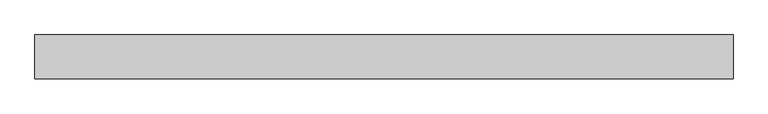
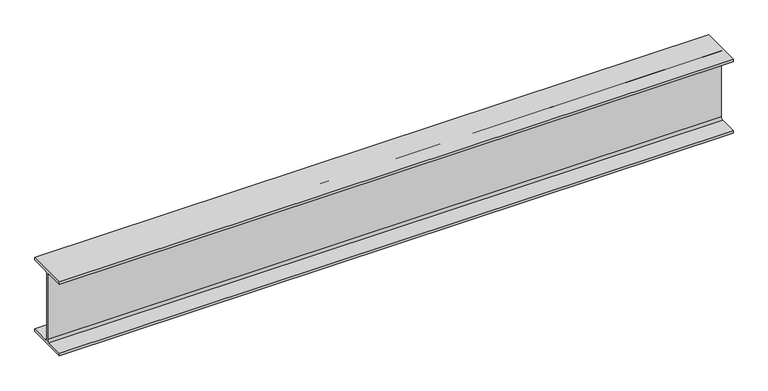
"""IFC4 building model written with IfcOpenShell, lengths in millimetres: beam geometry, Old_Steel Beam_H-KSD3502 : H_SB_ASB_H-194×150x6x9."""

import ifcopenshell
import ifcopenshell.guid

model = None  # the IFC model being written
_history = None  # IfcOwnerHistory: only IFC2X3 demands one
_inside = {}  # id of a spatial element -> (the spatial element, [elements in it])
_under = {}  # id of a project, library or spatial element -> (it, [spatial elements below it])
_declared = {}  # id of a project -> (the project, [libraries it declares])
_typed = {}  # id of a type object -> (the type object, [elements of that type])
_made_of = {}  # id of a material, layer set ... -> (it, [elements and type objects made of it])


def new_model(schema):
    """Start an empty IFC model of exactly this schema.

    Asked for "IFC4X3", IfcOpenShell would pick the latest addendum, in which some entities
    have other attributes; the version numbers below select the first issue.
    IFC2X3 requires an IfcOwnerHistory on every rooted entity: one is made here for all.
    """
    global model, _history
    if schema == "IFC4X3":
        model = ifcopenshell.file(schema_version=(4, 3, 0, 0))
    else:
        model = ifcopenshell.file(schema=schema)
    _inside.clear()
    _under.clear()
    _declared.clear()
    _typed.clear()
    _made_of.clear()
    _history = None
    if model.schema == "IFC2X3":
        org = make("IfcOrganization", Name="unknown")
        user = make(
            "IfcPersonAndOrganization",
            ThePerson=make("IfcPerson", FamilyName="unknown"),
            TheOrganization=org,
        )
        app = make(
            "IfcApplication",
            ApplicationDeveloper=org,
            Version="unknown",
            ApplicationFullName="unknown",
            ApplicationIdentifier="unknown",
        )
        _history = make(
            "IfcOwnerHistory",
            OwningUser=user,
            OwningApplication=app,
            ChangeAction="ADDED",
            CreationDate=0,
        )
    return model


def make(cls, **values):
    """One entity of the class cls with the attributes given. An attribute that is None is left unset."""
    return model.create_entity(
        cls, **{name: value for name, value in values.items() if value is not None}
    )


def rooted(cls, **values):
    """An entity with a GlobalId (a new one), such as an element, a storey or a relation."""
    return make(cls, GlobalId=ifcopenshell.guid.new(), OwnerHistory=_history, **values)


def si_unit(unit_type, name, prefix=None):
    """IfcSIUnit, for example si_unit("LENGTHUNIT", "METRE", prefix="MILLI")."""
    return make("IfcSIUnit", UnitType=unit_type, Prefix=prefix, Name=name)


def assignment(units):
    """IfcUnitAssignment: the units of a project."""
    return None if units is None else make("IfcUnitAssignment", Units=units)


def point(xyz):
    """IfcCartesianPoint."""
    return None if xyz is None else make("IfcCartesianPoint", Coordinates=xyz)


def direction(xyz):
    """IfcDirection."""
    return None if xyz is None else make("IfcDirection", DirectionRatios=xyz)


def frame(location, z_axis=None, x_axis=None):
    """IfcAxis2Placement3D, a coordinate frame: its origin and axes. An axis left out is left unset."""
    return make(
        "IfcAxis2Placement3D",
        Location=point(location),
        Axis=direction(z_axis),
        RefDirection=direction(x_axis),
    )


def frame_2d(location, x_axis=None):
    """IfcAxis2Placement2D, a coordinate frame in the plane: its origin and x axis."""
    return make(
        "IfcAxis2Placement2D", Location=point(location), RefDirection=direction(x_axis)
    )


def origin():
    """The frame at (0, 0, 0) with its axes left unset."""
    return frame((0.0, 0.0, 0.0))


def place(relative_to, where):
    """IfcLocalPlacement: puts the frame where relative to a parent placement (None: the world)."""
    return make(
        "IfcLocalPlacement", PlacementRelTo=relative_to, RelativePlacement=where
    )


def context(
    kind, dimensions, precision=None, world=None, true_north=None, identifier=None
):
    """IfcGeometricRepresentationContext, for example the 3D "Model" context."""
    return make(
        "IfcGeometricRepresentationContext",
        ContextIdentifier=identifier,
        ContextType=kind,
        CoordinateSpaceDimension=dimensions,
        Precision=precision,
        WorldCoordinateSystem=world,
        TrueNorth=true_north,
    )


def project(units=None, contexts=None):
    """IfcProject with its units and contexts."""
    return rooted(
        "IfcProject",
        Name="project",
        RepresentationContexts=contexts,
        UnitsInContext=assignment(units),
    )


def spatial(cls, under=None, at=None, **own):
    """A site, building, storey or space (cls), placed at a placement, below another one or the project."""
    s = rooted(cls, ObjectPlacement=at, **own)
    if under is not None:
        _under.setdefault(under.id(), (under, []))[1].append(s)
    return s


def polyline(points):
    """IfcPolyline through the points."""
    return make("IfcPolyline", Points=[point(p) for p in points])


def circle_curve(where, radius):
    """IfcCircle in the frame where."""
    return make("IfcCircle", Position=where, Radius=radius)


def trimmed(basis, trim1, trim2, sense, master):
    """IfcTrimmedCurve: the piece of a basis curve between two trims."""
    return make(
        "IfcTrimmedCurve",
        BasisCurve=basis,
        Trim1=trim1,
        Trim2=trim2,
        SenseAgreement=sense,
        MasterRepresentation=master,
    )


def segment(curve, same_sense, transition):
    """IfcCompositeCurveSegment."""
    return make(
        "IfcCompositeCurveSegment",
        Transition=transition,
        SameSense=same_sense,
        ParentCurve=curve,
    )


def composite_curve(segments, self_intersect=None):
    """IfcCompositeCurve: segments joined end to end."""
    return make("IfcCompositeCurve", Segments=segments, SelfIntersect=self_intersect)


def outline(outer, holes=None, kind="AREA"):
    """IfcArbitraryClosedProfileDef: a profile drawn as a closed curve; with holes, ...WithVoids."""
    if holes is None:
        return make("IfcArbitraryClosedProfileDef", ProfileType=kind, OuterCurve=outer)
    return make(
        "IfcArbitraryProfileDefWithVoids",
        ProfileType=kind,
        OuterCurve=outer,
        InnerCurves=holes,
    )


def extrude(swept, where, along, depth):
    """IfcExtrudedAreaSolid: the profile swept, set in the frame where, extruded along a direction by depth."""
    return make(
        "IfcExtrudedAreaSolid",
        SweptArea=swept,
        Position=where,
        ExtrudedDirection=direction(along),
        Depth=depth,
    )


def shape(context_of_items, identifier, shape_type, items):
    """IfcShapeRepresentation: the items that make up one representation, for example the "Body"."""
    return make(
        "IfcShapeRepresentation",
        ContextOfItems=context_of_items,
        RepresentationIdentifier=identifier,
        RepresentationType=shape_type,
        Items=items,
    )


def source(mapping_origin, context_of_items, identifier, shape_type, items):
    """IfcRepresentationMap: a shape defined once, which mapped items show again and again."""
    return make(
        "IfcRepresentationMap",
        MappingOrigin=mapping_origin,
        MappedRepresentation=shape(context_of_items, identifier, shape_type, items),
    )


def transform(
    local_origin,
    x_axis=None,
    y_axis=None,
    z_axis=None,
    scale=None,
    scale2=None,
    scale3=None,
    uniform=True,
):
    """IfcCartesianTransformationOperator3D, or its non-uniform kind. x_axis, y_axis, z_axis: its Axis1, 2, 3."""
    if uniform:
        return make(
            "IfcCartesianTransformationOperator3D",
            Axis1=direction(x_axis),
            Axis2=direction(y_axis),
            LocalOrigin=point(local_origin),
            Scale=scale,
            Axis3=direction(z_axis),
        )
    return make(
        "IfcCartesianTransformationOperator3DnonUniform",
        Axis1=direction(x_axis),
        Axis2=direction(y_axis),
        LocalOrigin=point(local_origin),
        Scale=scale,
        Axis3=direction(z_axis),
        Scale2=scale2,
        Scale3=scale3,
    )


def mapped(mapping_source, mapping_target):
    """IfcMappedItem: shows the shape of a source again, moved by a transform."""
    return make(
        "IfcMappedItem", MappingSource=mapping_source, MappingTarget=mapping_target
    )


def made_of(thing, what):
    """Note that an element or type object is made of a material, layer set ...; save() writes the relation."""
    if what is not None:
        _made_of.setdefault(what.id(), (what, []))[1].append(thing)
    return thing


def element(
    cls,
    number,
    at=None,
    inside=None,
    cuts=None,
    type_object=None,
    material=None,
    context=None,
    identifier="Body",
    shape_type=None,
    held_by="IfcProductDefinitionShape",
    body=None,
    shapes=None,
    **own,
):
    """One element of the class cls, such as IfcWall. Its Tag is "e" and its number.

    at: its placement. inside: the storey or other place that contains it. cuts: it is an
    opening in that element (IfcRelVoidsElement). A single representation is given by context,
    identifier, shape_type and body (its items); several are given by shapes. held_by: the class
    of the entity that holds the representations. save() writes the other relations.
    """
    e = rooted(cls, Tag="e%d" % number, ObjectPlacement=at, **own)
    if body is not None:
        shapes = [shape(context, identifier, shape_type, body)]
    if shapes is not None:
        e.Representation = make(held_by, Representations=shapes)
    if inside is not None:
        _inside.setdefault(inside.id(), (inside, []))[1].append(e)
    if cuts is not None:
        rooted(
            "IfcRelVoidsElement", RelatingBuildingElement=cuts, RelatedOpeningElement=e
        )
    if type_object is not None:
        _typed.setdefault(type_object.id(), (type_object, []))[1].append(e)
    return made_of(e, material)


def aggregate(whole, parts):
    """IfcRelAggregates: a whole, such as a stair, and the parts it consists of."""
    return rooted("IfcRelAggregates", RelatingObject=whole, RelatedObjects=parts)


def save(model, path):
    """Write the relations noted so far, then the file.

    IfcRelAggregates (storeys below a building ...), IfcRelContainedInSpatialStructure (elements
    in a storey), IfcRelDefinesByType, IfcRelAssociatesMaterial and IfcRelDeclares: one each for
    every whole, place, type object, material and project.
    """
    for whole, parts in _under.values():
        aggregate(whole, parts)
    for where, things in _inside.values():
        rooted(
            "IfcRelContainedInSpatialStructure",
            RelatedElements=things,
            RelatingStructure=where,
        )
    for kind, things in _typed.values():
        rooted("IfcRelDefinesByType", RelatedObjects=things, RelatingType=kind)
    for what, things in _made_of.values():
        rooted("IfcRelAssociatesMaterial", RelatedObjects=things, RelatingMaterial=what)
    for by, libraries in _declared.values():
        rooted("IfcRelDeclares", RelatingContext=by, RelatedDefinitions=libraries)
    model.write(path)


def beam_e9c9c49d(model_context):
    return source(origin(), model_context, "Body", "SweptSolid", [
        extrude(outline(composite_curve([segment(polyline([(82.5, -141.5), (82.5, -151.7), (-82.5, -151.7), (-82.5, -141.5), (-11.9, -141.5)]), True, "CONTINUOUS"), segment(trimmed(circle_curve(frame_2d((-11.9, -132.6)), 8.9), [point((-11.9, -141.5))], [point((-3.0, -132.6))], True, "CARTESIAN"), True, "CONTINUOUS"), segment(polyline([(-3.0, -132.6), (-3.0, 132.6)]), True, "CONTINUOUS"), segment(trimmed(circle_curve(frame_2d((-11.9, 132.6)), 8.9), [point((-3.0, 132.6))], [point((-11.9, 141.5))], True, "CARTESIAN"), True, "CONTINUOUS"), segment(polyline([(-11.9, 141.5), (-82.5, 141.5), (-82.5, 151.7), (82.5, 151.7), (82.5, 141.5), (11.9, 141.5)]), True, "CONTINUOUS"), segment(trimmed(circle_curve(frame_2d((11.9, 132.6)), 8.9), [point((11.9, 141.5))], [point((3.0, 132.6))], True, "CARTESIAN"), True, "CONTINUOUS"), segment(polyline([(3.0, 132.6), (3.0, -132.6)]), True, "CONTINUOUS"), segment(trimmed(circle_curve(frame_2d((11.9, -132.6)), 8.9), [point((3.0, -132.6))], [point((11.9, -141.5))], True, "CARTESIAN"), True, "CONTINUOUS"), segment(polyline([(11.9, -141.5), (82.5, -141.5)]), True, "CONTINUOUS")], self_intersect=False)), frame((-1068.0314701, 0.0, 0.0), z_axis=(1.0, 0.0, 0.0), x_axis=(0.0, 1.0, 0.0)), (0.0, 0.0, 1.0), 2617.0588612),
    ])


if __name__ == "__main__":
    model = new_model("IFC4")
    model_context = context("Model", 3, world=origin())
    ifc_project = project(units=[si_unit("LENGTHUNIT", "METRE", prefix="MILLI")], contexts=[model_context])
    site = spatial("IfcSite", under=ifc_project)
    building = spatial("IfcBuilding", under=site)
    placement = place(None, origin())
    beam_shape = beam_e9c9c49d(model_context)
    element("IfcBeam", 1, ObjectType="Old_Steel Beam_H-KSD3502 : H_SB_ASB_H-194×150x6x9", at=placement, inside=building, context=model_context, shape_type="MappedRepresentation", body=[
        mapped(beam_shape, transform((0.0, 0.0, 0.0), x_axis=(1.0, 0.0, 0.0), y_axis=(0.0, 1.0, 0.0), z_axis=(0.0, 0.0, 1.0))),
    ])
    save(model, "model.ifc")

# Revit data of these elements
# Type "Old_Steel Beam_H-KSD3502 : H_SB_ASB_H-194×150x6x9"
#   Width = 15.0 cm
#   Web Thickness = 0.6 cm
#   Web Fillet = 1.3 cm
#   Warping Constant = 43316.0 cm⁶
#   Torsional Moment of Inertia = 8.622 cm⁴
#   Torsional Modulus = 1.0 cm³
#   Section Area = 39.01 cm²
#   Plastic Modulus weak axis = 104.0 cm³
#   Plastic Modulus strong axis = 309.0 cm³
#   Perimeter = 0.95 m²/m
#   Nominal Weight = 30.60 kgf/m
#   Moment of Inertia weak axis = 507.00 cm⁴
#   Moment of Inertia strong axis = 2690.00 cm⁴
#   Height = 19.4 cm
#   Flange Thickness = 0.9 cm
#   Elastic Modulus weak axis = 67.6 cm³
#   Elastic Modulus strong axis = 277.0 cm³
#   Centroid Vertical = 9.7 cm
#   Centroid Horizontal = 7.5 cm
#   Length [instance default] = 1.5240 m
#   Structural Material [instance default] = Steel, 45-345
#   Assembly Code = ""
# Element 1 (IfcBeam, "Old_Steel Beam_H-KSD3502 : H_SB_ASB_H-194×150x6x9")
#   Structural Material = none
# Materials
#   "Steel, 45-345": class "Metal", colour RGB 189 187 185, transparency 0, Description = "Steel 345 MPa", Cost = 0
